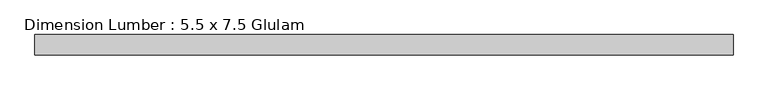
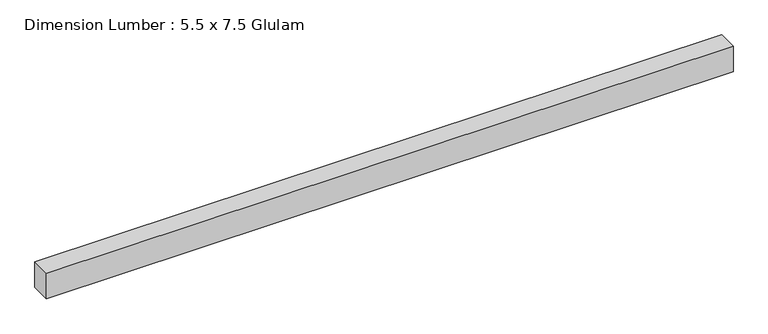
"""IFC4 building model written with IfcOpenShell, lengths in millimetres: beam geometry, Dimension Lumber : 5.5 x 7.5 Glulam."""

from ifc_helpers import new_model, si_unit, frame, origin, place, context, project, spatial, polyline, outline, extrude, source, transform, mapped, element, save


def dimension_lumber_5_5_x_7_5_glulam_5a1f9f63(model_context):
    return source(origin(), model_context, "Body", "SweptSolid", [
        extrude(outline(polyline([(2439.95575, 69.85), (2439.95575, -69.85), (-2389.02875, -69.85), (-2389.02875, 69.85), (2439.95575, 69.85)])), frame((0.0, 0.0, -95.25), z_axis=(0.0, 0.0, 1.0), x_axis=(1.0, 0.0, 0.0)), (0.0, 0.0, 1.0), 190.5),
    ])


if __name__ == "__main__":
    model = new_model("IFC4")
    model_context = context("Model", 3, world=origin())
    ifc_project = project(units=[si_unit("LENGTHUNIT", "METRE", prefix="MILLI")], contexts=[model_context])
    site = spatial("IfcSite", under=ifc_project)
    building = spatial("IfcBuilding", under=site)
    placement = place(None, origin())
    dimension_lumber_5_5_x_7_5_glulam_shape = dimension_lumber_5_5_x_7_5_glulam_5a1f9f63(model_context)
    element("IfcBeam", 1, ObjectType="Dimension Lumber : 5.5 x 7.5 Glulam", at=placement, inside=building, context=model_context, shape_type="MappedRepresentation", body=[
        mapped(dimension_lumber_5_5_x_7_5_glulam_shape, transform((0.0, 0.0, 0.0), x_axis=(1.0, 0.0, 0.0), y_axis=(0.0, 1.0, 0.0), z_axis=(0.0, 0.0, 1.0))),
    ])
    save(model, "model.ifc")

# Revit data of these elements
# Type "Dimension Lumber : 5.5 x 7.5 Glulam"
#   Keynote = "M06181300.01"
#   Assembly Code = "B10"
#   A = 0.0755556 SF
#   Length [instance default] = 5' - 0"
#   b = 0' - 5 1/2"
#   d = 0' - 7 1/2"
#   Structural Material [instance default] = Softwood, Lumber
# Element 1 (IfcBeam, "Dimension Lumber : 5.5 x 7.5 Glulam")
#   Structural Material = 5 1/2" X 7 1/2" EXTERIOR GRADE GLULAM BEAMS
#   Materials on its faces: "5 1/2\" X 7 1/2\" EXTERIOR GRADE GLULAM BEAMS"
# Materials
#   "Softwood, Lumber": class "Wood", colour RGB 212 179 113, transparency 0, Description = "Pinus Echinata", Cost = 0
#   "5 1/2\" X 7 1/2\" EXTERIOR GRADE GLULAM BEAMS": class "Wood", colour RGB 212 179 113, transparency 0, Description = "Pinus Echinata", Cost = 0
